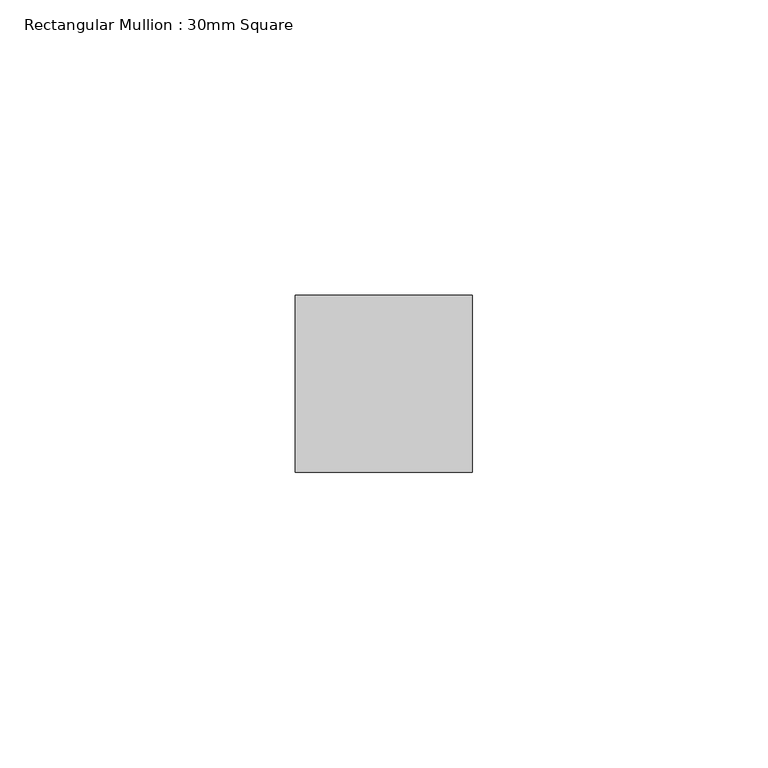
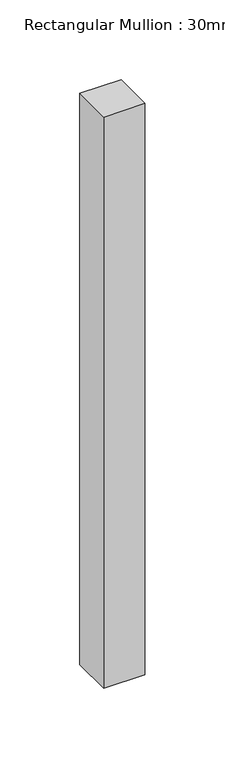
"""IFC4 building model written with IfcOpenShell, lengths in millimetres: member geometry, Rectangular Mullion : 30mm Square."""

from ifc_helpers import new_model, si_unit, frame, origin, place, context, project, spatial, polyline, outline, extrude, source, transform, mapped, element, save


def rectangular_mullion_30mm_square_d9e325f0(model_context):
    return source(origin(), model_context, "Body", "SweptSolid", [
        extrude(outline(polyline([(15.0, 15.0), (15.0, -15.0), (-15.0, -15.0), (-15.0, 15.0), (15.0, 15.0)])), frame((0.0, 0.0, -437.605017), z_axis=(0.0, 0.0, 1.0), x_axis=(1.0, 0.0, 0.0)), (0.0, 0.0, 1.0), 437.605017),
    ])


if __name__ == "__main__":
    model = new_model("IFC4")
    model_context = context("Model", 3, world=origin())
    ifc_project = project(units=[si_unit("LENGTHUNIT", "METRE", prefix="MILLI")], contexts=[model_context])
    site = spatial("IfcSite", under=ifc_project)
    building = spatial("IfcBuilding", under=site)
    placement = place(None, origin())
    rectangular_mullion_30mm_square_shape = rectangular_mullion_30mm_square_d9e325f0(model_context)
    element("IfcMember", 1, ObjectType="Rectangular Mullion : 30mm Square", at=placement, inside=building, context=model_context, shape_type="MappedRepresentation", body=[
        mapped(rectangular_mullion_30mm_square_shape, transform((0.0, 0.0, 0.0), x_axis=(1.0, 0.0, 0.0), y_axis=(0.0, 1.0, 0.0), z_axis=(0.0, 0.0, 1.0))),
    ])
    save(model, "model.ifc")

# Revit data of these elements
# Type "Rectangular Mullion : 30mm Square"
#   built-in parameter 1007304 = 0.0984252 (stored number, unit not read)
#   built-in parameter 1007301 = 0.0492126 (stored number, unit not read)
#   built-in parameter 1007300 = 0.0492126 (stored number, unit not read)
# Element 1 (IfcMember, "Rectangular Mullion : 30mm Square")
#   Materials on its faces: "Aluminum"
# Materials
#   "Aluminum": class "Metal", colour RGB 244 244 244, transparency 0, Description = "Aluminum 6061", Cost = 0
